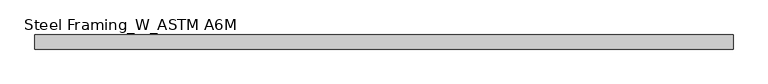
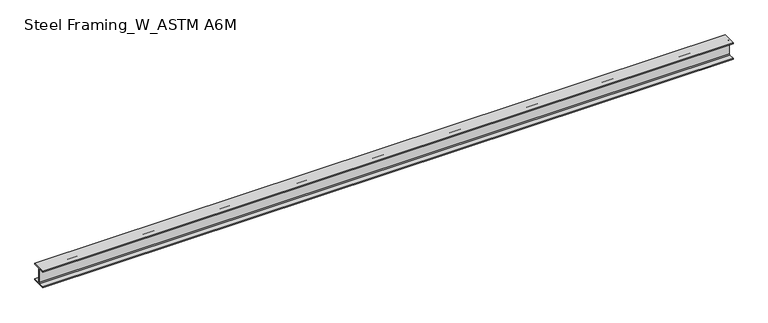
"""IFC4 building model written with IfcOpenShell, lengths in millimetres: beam geometry, Steel Framing_W_ASTM A6M : H_SB_AR_S02_W250x49.1_RB3."""

from ifc_helpers import new_model, si_unit, point, frame, frame_2d, origin, place, context, project, spatial, polyline, circle_curve, trimmed, segment, composite_curve, outline, extrude, source, transform, mapped, element, save


def steel_framing_w_astm_a6m_b181222c(model_context):
    return source(origin(), model_context, "Body", "SweptSolid", [
        extrude(outline(composite_curve([segment(polyline([(101.0, -112.5), (101.0, -123.5), (-101.0, -123.5), (-101.0, -112.5), (-16.385, -112.5)]), True, "CONTINUOUS"), segment(trimmed(circle_curve(frame_2d((-16.385, -99.8)), 12.7), [point((-16.385, -112.5))], [point((-3.685, -99.8))], True, "CARTESIAN"), True, "CONTINUOUS"), segment(polyline([(-3.685, -99.8), (-3.685, 99.8)]), True, "CONTINUOUS"), segment(trimmed(circle_curve(frame_2d((-16.385, 99.8)), 12.7), [point((-3.685, 99.8))], [point((-16.385, 112.5))], True, "CARTESIAN"), True, "CONTINUOUS"), segment(polyline([(-16.385, 112.5), (-101.0, 112.5), (-101.0, 123.5), (101.0, 123.5), (101.0, 112.5), (16.385, 112.5)]), True, "CONTINUOUS"), segment(trimmed(circle_curve(frame_2d((16.385, 99.8)), 12.7), [point((16.385, 112.5))], [point((3.685, 99.8))], True, "CARTESIAN"), True, "CONTINUOUS"), segment(polyline([(3.685, 99.8), (3.685, -99.8)]), True, "CONTINUOUS"), segment(trimmed(circle_curve(frame_2d((16.385, -99.8)), 12.7), [point((3.685, -99.8))], [point((16.385, -112.5))], True, "CARTESIAN"), True, "CONTINUOUS"), segment(polyline([(16.385, -112.5), (101.0, -112.5)]), True, "CONTINUOUS")], self_intersect=False)), frame((-4987.2, 0.0, 0.0), z_axis=(1.0, 0.0, 0.0), x_axis=(0.0, 1.0, 0.0)), (0.0, 0.0, 1.0), 9974.4),
    ])


if __name__ == "__main__":
    model = new_model("IFC4")
    model_context = context("Model", 3, world=origin())
    ifc_project = project(units=[si_unit("LENGTHUNIT", "METRE", prefix="MILLI")], contexts=[model_context])
    site = spatial("IfcSite", under=ifc_project)
    building = spatial("IfcBuilding", under=site)
    placement = place(None, origin())
    steel_framing_w_astm_a6m_shape = steel_framing_w_astm_a6m_b181222c(model_context)
    element("IfcBeam", 1, ObjectType="Steel Framing_W_ASTM A6M : H_SB_AR_S02_W250x49.1_RB3", at=placement, inside=building, context=model_context, shape_type="MappedRepresentation", body=[
        mapped(steel_framing_w_astm_a6m_shape, transform((0.0, 0.0, 0.0), x_axis=(1.0, 0.0, 0.0), y_axis=(0.0, 1.0, 0.0), z_axis=(0.0, 0.0, 1.0))),
    ])
    save(model, "model.ifc")

# Revit data of these elements
# Type "Steel Framing_W_ASTM A6M : H_SB_AR_S02_W250x49.1_RB3"
#   Type Mark = "RB3"
#   Section Name Key = "W10x33"
#   Width = 20.2 cm
#   Web Thickness = 0.737 cm
#   Web Fillet = 1.27 cm
#   Warping Constant = 212000.0 cm⁶
#   Torsional Moment of Inertia = 24.30 cm⁴
#   Section Area = 62.6 cm²
#   Plastic Modulus weak axis = 229.0 cm³
#   Plastic Modulus strong axis = 636.0 cm³
#   Perimeter = 1.27 m²/m
#   Nominal Weight = 49.10 kgf/m
#   Moment of Inertia weak axis = 1520.00 cm⁴
#   Moment of Inertia strong axis = 7120.00 cm⁴
#   Height = 24.7 cm
#   Flange Thickness = 1.1 cm
#   Elastic Modulus weak axis = 151.0 cm³
#   Elastic Modulus strong axis = 574.0 cm³
#   Centroid Vertical = 12.35 cm
#   Centroid Horizontal = 10.1 cm
#   Length [instance default] = 1500 mm
#   Structural Material [instance default] = Steel, 45-345
#   Bolt Spacing = 0
#   Assembly Code = ""
# Element 1 (IfcBeam, "Steel Framing_W_ASTM A6M : H_SB_AR_S02_W250x49.1_RB3")
#   Materials on its faces: "Steel, 45-345"
# Materials
#   "Steel, 45-345": class "Metal", colour RGB 189 187 185, transparency 0, Description = "Steel 345 MPa", Cost = 0
